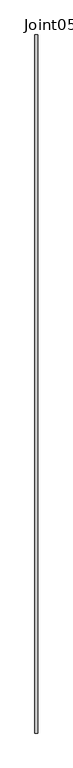
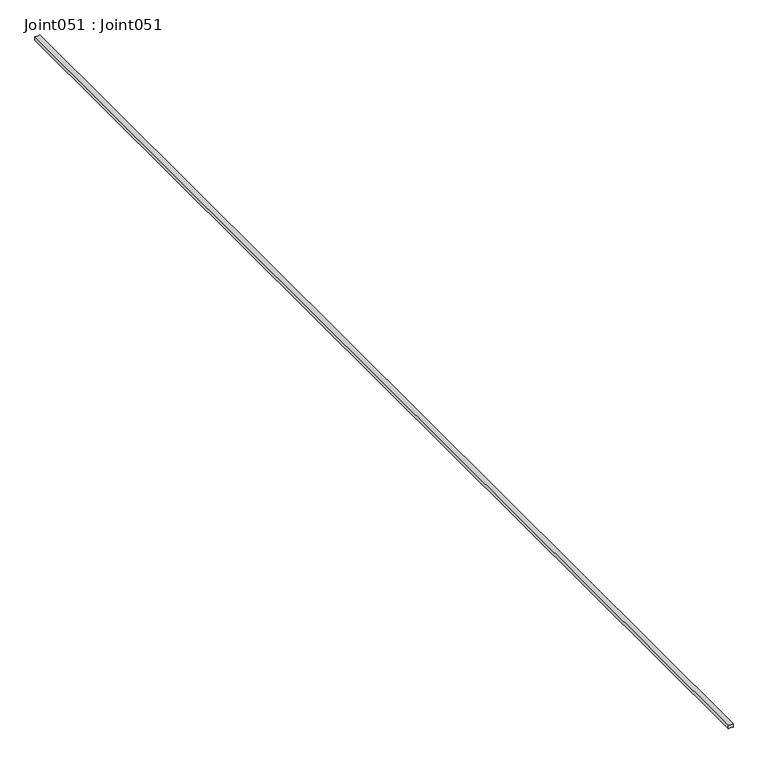
"""IFC4 building model written with IfcOpenShell, lengths in millimetres: proxy geometry, Joint051 : Joint051."""

from ifc_helpers import new_model, si_unit, point, frame, frame_2d, origin, place, context, project, spatial, polyline, circle_curve, trimmed, segment, composite_curve, outline, extrude, source, transform, mapped, element, save


def joint051_joint051_deac0ab0(model_context):
    return source(origin(), model_context, "Body", "SweptSolid", [
        extrude(outline(composite_curve([segment(trimmed(circle_curve(frame_2d((43727.3490074, 6175.5624116)), 9.8007347), [point((43736.2517817, 6171.4642399))], [point((43736.2517817, 6179.6605833))], True, "CARTESIAN"), True, "CONTINUOUS"), segment(polyline([(43736.2517817, 6179.6605833), (43742.7041053, 6179.6605833)]), True, "CONTINUOUS"), segment(trimmed(circle_curve(frame_2d((43750.4055009, 6175.5624116)), 8.7239042), [point((43742.7041053, 6179.6605833))], [point((43742.7041053, 6171.4642399))], True, "CARTESIAN"), True, "CONTINUOUS"), segment(polyline([(43742.7041053, 6171.4642399), (43736.2517817, 6171.4642399)]), True, "CONTINUOUS")], self_intersect=False)), frame((0.0, -1052.891, 0.0), z_axis=(0.0, 1.0, 0.0), x_axis=(0.0, 0.0, 1.0)), (0.0, 0.0, 1.0), 2000.0),
    ])


if __name__ == "__main__":
    model = new_model("IFC4")
    model_context = context("Model", 3, world=origin())
    ifc_project = project(units=[si_unit("LENGTHUNIT", "METRE", prefix="MILLI")], contexts=[model_context])
    site = spatial("IfcSite", under=ifc_project)
    building = spatial("IfcBuilding", under=site)
    placement = place(None, origin())
    joint051_joint051_shape = joint051_joint051_deac0ab0(model_context)
    element("IfcBuildingElementProxy", 1, Name="Joint051 : Joint051", ObjectType="Joint051 : Joint051", at=placement, inside=building, context=model_context, shape_type="MappedRepresentation", body=[
        mapped(joint051_joint051_shape, transform((0.0, 0.0, 0.0), x_axis=(1.0, 0.0, 0.0), y_axis=(0.0, 1.0, 0.0), z_axis=(0.0, 0.0, 1.0))),
    ])
    save(model, "model.ifc")

# Revit data of these elements
# Type "Joint051 : Joint051"
#   NameOverride = "Joint051"
# Element 1 (IfcBuildingElementProxy, "Joint051 : Joint051")
#   Materials on its faces: "SEALANT"
# Materials
#   "SEALANT": class "Unassigned", colour RGB 142 225 148, transparency 0
